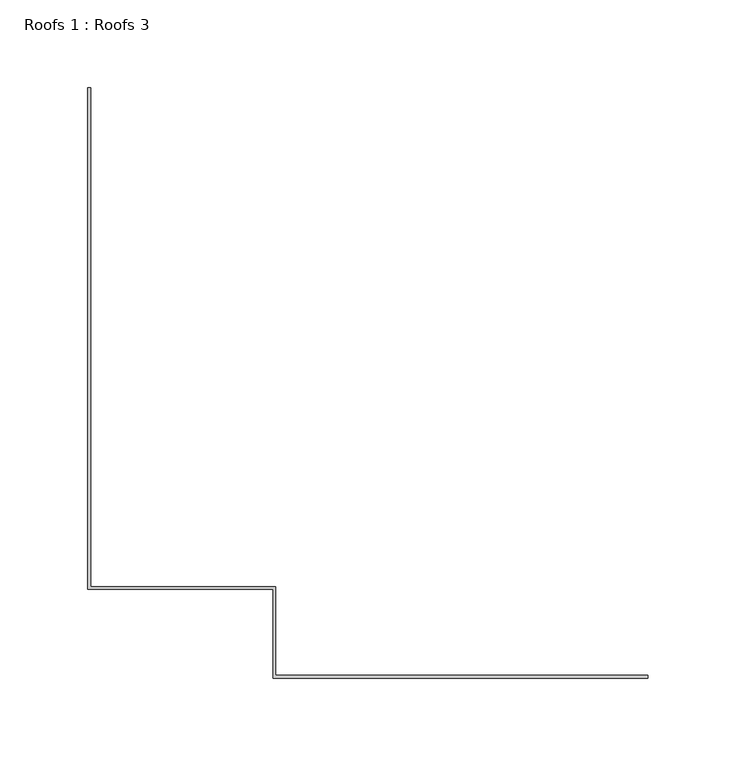
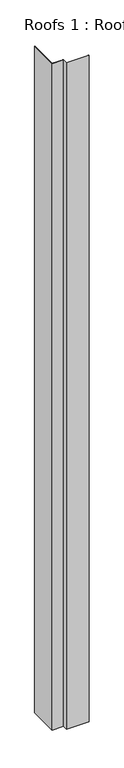
"""IFC4 building model written with IfcOpenShell, lengths in millimetres: proxy geometry, Roofs 1 : Roofs 3."""

from ifc_helpers import new_model, si_unit, frame, origin, place, context, project, spatial, polyline, outline, extrude, source, transform, mapped, element, save


def roofs_1_roofs_3_b891b27c(model_context):
    return source(origin(), model_context, "Body", "SweptSolid", [
        extrude(outline(polyline([(23408.3286726, 25862.8006531), (23409.9161726, 25862.8006531), (23409.9161726, 25578.9745393), (23515.3617059, 25578.9745393), (23515.3617059, 25528.4469112), (23727.2929559, 25528.4469112), (23727.2929559, 25526.8594112), (23513.7742059, 25526.8594112), (23513.7742059, 25577.3870393), (23408.3286726, 25577.3870393), (23408.3286726, 25862.8006531)])), frame((0.0, 0.0, 265582.8945751), z_axis=(0.0, 0.0, 1.0), x_axis=(1.0, 0.0, 0.0)), (0.0, 0.0, 1.0), 6636.6392074),
    ])


if __name__ == "__main__":
    model = new_model("IFC4")
    model_context = context("Model", 3, world=origin())
    ifc_project = project(units=[si_unit("LENGTHUNIT", "METRE", prefix="MILLI")], contexts=[model_context])
    site = spatial("IfcSite", under=ifc_project)
    building = spatial("IfcBuilding", under=site)
    placement = place(None, origin())
    roofs_1_roofs_3_shape = roofs_1_roofs_3_b891b27c(model_context)
    element("IfcBuildingElementProxy", 1, Name="Roofs 1 : Roofs 3", ObjectType="Roofs 1 : Roofs 3", at=placement, inside=building, context=model_context, shape_type="MappedRepresentation", body=[
        mapped(roofs_1_roofs_3_shape, transform((0.0, 0.0, 0.0), x_axis=(1.0, 0.0, 0.0), y_axis=(0.0, 1.0, 0.0), z_axis=(0.0, 0.0, 1.0))),
    ])
    save(model, "model.ifc")

# Revit data of these elements
# Element 1 (IfcBuildingElementProxy, "Roofs 1 : Roofs 3")
#   Materials on its faces: "UV STABLE WATER RESISTANT VAPOR PERMEABLE AIR BARRIER (WRVPAB) - WRAP JAMBS/HEADERS - BLACK COLOR"
# Materials
#   "UV STABLE WATER RESISTANT VAPOR PERMEABLE AIR BARRIER (WRVPAB) - WRAP JAMBS/HEADERS - BLACK COLOR": class "Generic", colour RGB 51 162 45, transparency 0, Description = "Polyethylene film membrane", Cost = 0
